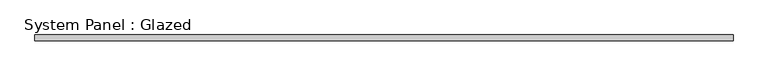
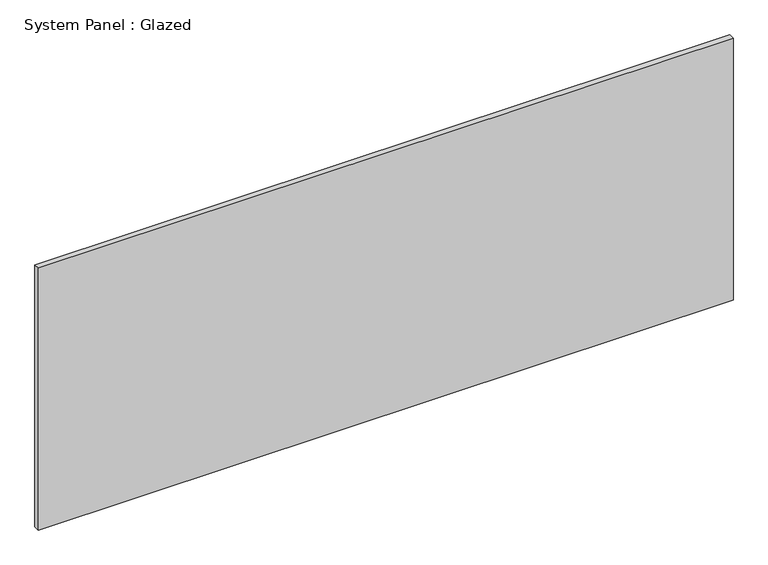
"""IFC4 building model written with IfcOpenShell, lengths in millimetres: plate geometry, System Panel : Glazed."""

from ifc_helpers import new_model, si_unit, origin, origin_with_axes, place, context, project, spatial, polyline, outline, extrude, source, transform, mapped, element, save


def system_panel_glazed_efb213d5(model_context):
    return source(origin(), model_context, "Body", "SweptSolid", [
        extrude(outline(polyline([(1524.0000002, 19.05), (-1524.0000002, 19.05), (-1524.0000002, 44.45), (1524.0000002, 44.45), (1524.0000002, 19.05)])), origin_with_axes(), (0.0, 0.0, 1.0), 1216.0),
    ])


if __name__ == "__main__":
    model = new_model("IFC4")
    model_context = context("Model", 3, world=origin())
    ifc_project = project(units=[si_unit("LENGTHUNIT", "METRE", prefix="MILLI")], contexts=[model_context])
    site = spatial("IfcSite", under=ifc_project)
    building = spatial("IfcBuilding", under=site)
    placement = place(None, origin())
    system_panel_glazed_shape = system_panel_glazed_efb213d5(model_context)
    element("IfcPlate", 1, ObjectType="System Panel : Glazed", at=placement, inside=building, context=model_context, shape_type="MappedRepresentation", body=[
        mapped(system_panel_glazed_shape, transform((0.0, 0.0, 0.0), x_axis=(1.0, 0.0, 0.0), y_axis=(0.0, 1.0, 0.0), z_axis=(0.0, 0.0, 1.0))),
    ])
    save(model, "model.ifc")

# Revit data of these elements
# Type "System Panel : Glazed"
#   Construction Type Id = "GSP4R"
#   Analytic Construction = "1/8 in Pilkington single glazing"
#   Visual Light Transmittance = 0.9
#   Solar Heat Gain Coefficient = 0.86
#   Heat Transfer Coefficient (U) = 6.7069 W/(m²·K)
# Element 1 (IfcPlate, "System Panel : Glazed")
#   Materials on its faces: "Glass"
# Materials
#   "Glass": class "Glass", colour RGB 0 128 192, transparency 0.75, Description = "Soda Lime Glass", Cost = 0
